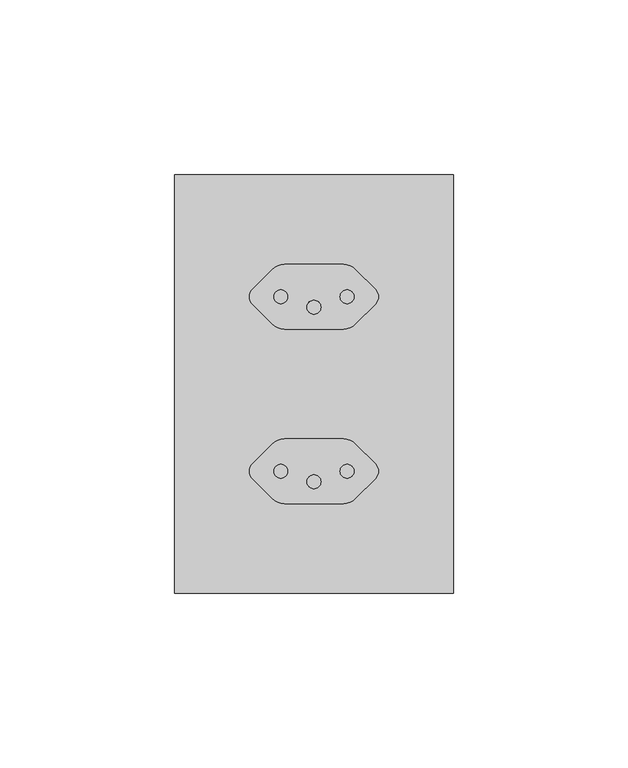
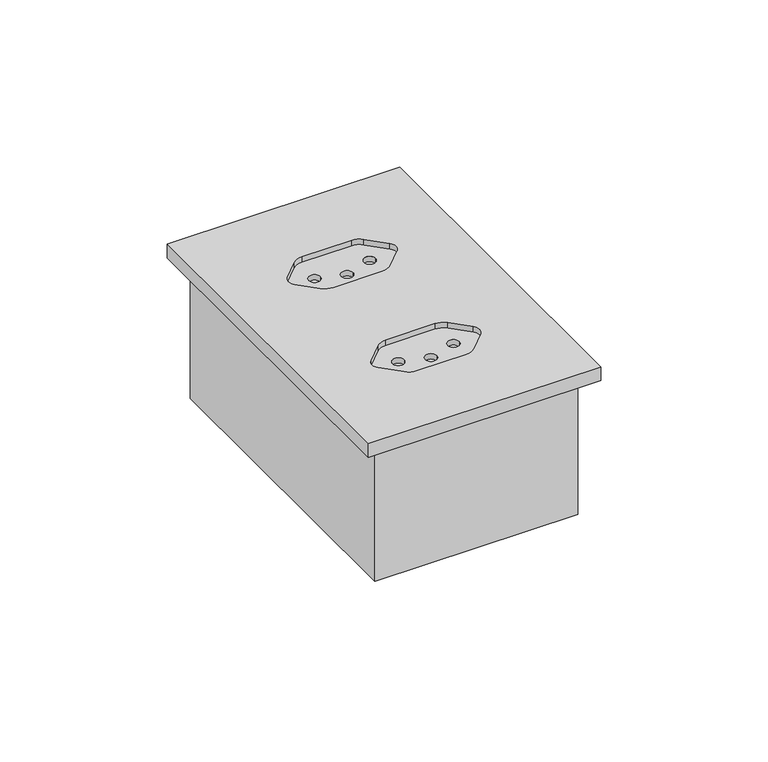
"""IFC4 building model written with IfcOpenShell, lengths in millimetres: proxy geometry, CAIXA VERTICE V7 : Tomada 10A 2s."""

from ifc_helpers import new_model, si_unit, frame, origin, place, context, project, spatial, polyline, circle_curve, faceted_brep, source, transform, mapped, element, save
from ifc_brep_helpers import plane_surface, revolved_surface, advanced_brep


def electrical_fixtures_dab928c3(model_context):
    return source(origin(), model_context, "Body", "SolidModel", [
        faceted_brep([(33.0, -1047.0, -48.0), (-33.0, -1047.0, -48.0), (-33.0, -1153.0, -48.0), (33.0, -1153.0, -48.0), (35.0, -1155.0, -50.0), (-35.0, -1155.0, -50.0), (-35.0, -1045.0, -50.0), (35.0, -1045.0, -50.0), (35.0, -1155.0, 0.0), (-35.0, -1155.0, 0.0), (-35.0, -1045.0, 0.0), (35.0, -1045.0, 0.0), (33.0, -1153.0, 0.0), (-33.0, -1153.0, 0.0), (-33.0, -1047.0, 0.0), (33.0, -1047.0, 0.0)], [[[0, 1, 2, 3]], [[4, 5, 6, 7]], [[4, 8, 9, 5]], [[9, 10, 6, 5]], [[10, 11, 7, 6]], [[11, 8, 4, 7]], [[8, 11, 10, 9], [12, 13, 14, 15]], [[15, 0, 3, 12]], [[14, 1, 0, 15]], [[13, 2, 1, 14]], [[12, 3, 2, 13]]]),
        advanced_brep(
        [(40.0, -1160.0, 5.0), (40.0, -1040.0, 5.0), (-40.0, -1040.0, 5.0), (-40.0, -1160.0, 5.0), (8.4215729, -1115.75, 5.0), (11.9571068, -1117.2144661, 5.0), (17.6213203, -1122.8786797, 5.0), (17.6213203, -1127.1213203, 5.0), (11.9571068, -1132.7855339, 5.0), (8.4215729, -1134.25, 5.0), (-8.4215729, -1134.25, 5.0), (-11.9571068, -1132.7855339, 5.0), (-17.6213203, -1127.1213203, 5.0), (-17.6213203, -1122.8786797, 5.0), (-11.9571068, -1117.2144661, 5.0), (-8.4215729, -1115.75, 5.0), (8.4215729, -1065.75, 5.0), (11.9571068, -1067.2144661, 5.0), (17.6213203, -1072.8786797, 5.0), (17.6213203, -1077.1213203, 5.0), (11.9571068, -1082.7855339, 5.0), (8.4215729, -1084.25, 5.0), (-8.4215729, -1084.25, 5.0), (-11.9571068, -1082.7855339, 5.0), (-17.6213203, -1077.1213203, 5.0), (-17.6213203, -1072.8786797, 5.0), (-11.9571068, -1067.2144661, 5.0), (-8.4215729, -1065.75, 5.0), (-40.0, -1160.0, 0.0), (-40.0, -1040.0, 0.0), (40.0, -1040.0, 0.0), (40.0, -1160.0, 0.0), (8.4215729, -1115.75, 3.0), (-8.4215729, -1115.75, 3.0), (-11.9571068, -1117.2144661, 3.0), (-17.6213203, -1122.8786797, 3.0), (-17.6213203, -1127.1213203, 3.0), (-11.9571068, -1132.7855339, 3.0), (-8.4215729, -1134.25, 3.0), (8.4215729, -1134.25, 3.0), (11.9571068, -1132.7855339, 3.0), (17.6213203, -1127.1213203, 3.0), (17.6213203, -1122.8786797, 3.0), (11.9571068, -1117.2144661, 3.0), (-7.5, -1125.0, 3.0), (-11.5, -1125.0, 3.0), (11.5, -1125.0, 3.0), (7.5, -1125.0, 3.0), (2.0, -1128.0, 3.0), (-2.0, -1128.0, 3.0), (-11.5, -1125.0, 1.0), (-7.5, -1125.0, 1.0), (7.5, -1125.0, 1.0), (11.5, -1125.0, 1.0), (-2.0, -1128.0, 1.0), (2.0, -1128.0, 1.0), (8.4215729, -1065.75, 3.0), (-8.4215729, -1065.75, 3.0), (-11.9571068, -1067.2144661, 3.0), (-17.6213203, -1072.8786797, 3.0), (-17.6213203, -1077.1213203, 3.0), (-11.9571068, -1082.7855339, 3.0), (-8.4215729, -1084.25, 3.0), (8.4215729, -1084.25, 3.0), (11.9571068, -1082.7855339, 3.0), (17.6213203, -1077.1213203, 3.0), (17.6213203, -1072.8786797, 3.0), (11.9571068, -1067.2144661, 3.0), (-7.5, -1075.0, 3.0), (-11.5, -1075.0, 3.0), (11.5, -1075.0, 3.0), (7.5, -1075.0, 3.0), (2.0, -1078.0, 3.0), (-2.0, -1078.0, 3.0), (-11.5, -1075.0, 1.0), (-7.5, -1075.0, 1.0), (7.5, -1075.0, 1.0), (11.5, -1075.0, 1.0), (-2.0, -1078.0, 1.0), (2.0, -1078.0, 1.0)],
        [
            (0, 1),
            (1, 2),
            (2, 3),
            (3, 0),
            (4, 5, circle_curve(frame((8.4215729, -1120.75, 5.0), z_axis=(0.0, 0.0, -1.0), x_axis=(-1.0, 0.0, 0.0)), 5.0)),
            (5, 6),
            (6, 7, circle_curve(frame((15.5, -1125.0, 5.0), z_axis=(0.0, 0.0, -1.0), x_axis=(-1.0, 0.0, 0.0)), 3.0)),
            (7, 8),
            (8, 9, circle_curve(frame((8.4215729, -1129.25, 5.0), z_axis=(0.0, 0.0, -1.0), x_axis=(-1.0, 0.0, 0.0)), 5.0)),
            (9, 10),
            (10, 11, circle_curve(frame((-8.4215729, -1129.25, 5.0), z_axis=(0.0, 0.0, -1.0), x_axis=(-1.0, 0.0, 0.0)), 5.0)),
            (11, 12),
            (12, 13, circle_curve(frame((-15.5, -1125.0, 5.0), z_axis=(0.0, 0.0, -1.0), x_axis=(-1.0, 0.0, 0.0)), 3.0)),
            (13, 14),
            (14, 15, circle_curve(frame((-8.4215729, -1120.75, 5.0), z_axis=(0.0, 0.0, -1.0), x_axis=(-1.0, 0.0, 0.0)), 5.0)),
            (15, 4),
            (16, 17, circle_curve(frame((8.4215729, -1070.75, 5.0), z_axis=(0.0, 0.0, -1.0), x_axis=(-1.0, 0.0, 0.0)), 5.0)),
            (17, 18),
            (18, 19, circle_curve(frame((15.5, -1075.0, 5.0), z_axis=(0.0, 0.0, -1.0), x_axis=(-1.0, 0.0, 0.0)), 3.0)),
            (19, 20),
            (20, 21, circle_curve(frame((8.4215729, -1079.25, 5.0), z_axis=(0.0, 0.0, -1.0), x_axis=(-1.0, 0.0, 0.0)), 5.0)),
            (21, 22),
            (22, 23, circle_curve(frame((-8.4215729, -1079.25, 5.0), z_axis=(0.0, 0.0, -1.0), x_axis=(-1.0, 0.0, 0.0)), 5.0)),
            (23, 24),
            (24, 25, circle_curve(frame((-15.5, -1075.0, 5.0), z_axis=(0.0, 0.0, -1.0), x_axis=(-1.0, 0.0, 0.0)), 3.0)),
            (25, 26),
            (26, 27, circle_curve(frame((-8.4215729, -1070.75, 5.0), z_axis=(0.0, 0.0, -1.0), x_axis=(-1.0, 0.0, 0.0)), 5.0)),
            (27, 16),
            (28, 29),
            (29, 30),
            (30, 31),
            (31, 28),
            (3, 28),
            (31, 0),
            (2, 29),
            (1, 30),
            (32, 33),
            (33, 34, circle_curve(frame((-8.4215729, -1120.75, 3.0), z_axis=(0.0, 0.0, 1.0), x_axis=(-1.0, 0.0, 0.0)), 5.0)),
            (34, 35),
            (35, 36, circle_curve(frame((-15.5, -1125.0, 3.0), z_axis=(0.0, 0.0, 1.0), x_axis=(-1.0, 0.0, 0.0)), 3.0)),
            (36, 37),
            (37, 38, circle_curve(frame((-8.4215729, -1129.25, 3.0), z_axis=(0.0, 0.0, 1.0), x_axis=(-1.0, 0.0, 0.0)), 5.0)),
            (38, 39),
            (39, 40, circle_curve(frame((8.4215729, -1129.25, 3.0), z_axis=(0.0, 0.0, 1.0), x_axis=(-1.0, 0.0, 0.0)), 5.0)),
            (40, 41),
            (41, 42, circle_curve(frame((15.5, -1125.0, 3.0), z_axis=(0.0, 0.0, 1.0), x_axis=(-1.0, 0.0, 0.0)), 3.0)),
            (42, 43),
            (43, 32, circle_curve(frame((8.4215729, -1120.75, 3.0), z_axis=(0.0, 0.0, 1.0), x_axis=(-1.0, 0.0, 0.0)), 5.0)),
            (44, 45, circle_curve(frame((-9.5, -1125.0, 3.0), z_axis=(0.0, 0.0, -1.0), x_axis=(1.0, -2.301812013077709e-12, 0.0)), 2.0)),
            (45, 44, circle_curve(frame((-9.5, -1125.0, 3.0), z_axis=(0.0, 0.0, -1.0), x_axis=(1.0, -2.301812013077709e-12, 0.0)), 2.0)),
            (46, 47, circle_curve(frame((9.5, -1125.0, 3.0), z_axis=(0.0, 0.0, -1.0), x_axis=(1.0, -2.301812013077709e-12, 0.0)), 2.0)),
            (47, 46, circle_curve(frame((9.5, -1125.0, 3.0), z_axis=(0.0, 0.0, -1.0), x_axis=(1.0, -2.301812013077709e-12, 0.0)), 2.0)),
            (48, 49, circle_curve(frame((0.0, -1128.0, 3.0), z_axis=(0.0, 0.0, -1.0), x_axis=(1.0, -2.301812013077709e-12, 0.0)), 2.0)),
            (49, 48, circle_curve(frame((0.0, -1128.0, 3.0), z_axis=(0.0, 0.0, -1.0), x_axis=(1.0, -2.301812013077709e-12, 0.0)), 2.0)),
            (32, 4),
            (15, 33),
            (14, 34),
            (13, 35),
            (12, 36),
            (11, 37),
            (10, 38),
            (9, 39),
            (8, 40),
            (7, 41),
            (6, 42),
            (5, 43),
            (50, 51, circle_curve(frame((-9.5, -1125.0, 1.0), z_axis=(0.0, 0.0, 1.0), x_axis=(1.0, -2.301812013077709e-12, 0.0)), 2.0)),
            (51, 50, circle_curve(frame((-9.5, -1125.0, 1.0), z_axis=(0.0, 0.0, 1.0), x_axis=(1.0, -2.301812013077709e-12, 0.0)), 2.0)),
            (52, 53, circle_curve(frame((9.5, -1125.0, 1.0), z_axis=(0.0, 0.0, 1.0), x_axis=(1.0, -2.301812013077709e-12, 0.0)), 2.0)),
            (53, 52, circle_curve(frame((9.5, -1125.0, 1.0), z_axis=(0.0, 0.0, 1.0), x_axis=(1.0, -2.301812013077709e-12, 0.0)), 2.0)),
            (54, 55, circle_curve(frame((0.0, -1128.0, 1.0), z_axis=(0.0, 0.0, 1.0), x_axis=(1.0, -2.301812013077709e-12, 0.0)), 2.0)),
            (55, 54, circle_curve(frame((0.0, -1128.0, 1.0), z_axis=(0.0, 0.0, 1.0), x_axis=(1.0, -2.301812013077709e-12, 0.0)), 2.0)),
            (45, 50),
            (51, 44),
            (47, 52),
            (53, 46),
            (49, 54),
            (55, 48),
            (56, 57),
            (57, 58, circle_curve(frame((-8.4215729, -1070.75, 3.0), z_axis=(0.0, 0.0, 1.0), x_axis=(-1.0, 0.0, 0.0)), 5.0)),
            (58, 59),
            (59, 60, circle_curve(frame((-15.5, -1075.0, 3.0), z_axis=(0.0, 0.0, 1.0), x_axis=(-1.0, 0.0, 0.0)), 3.0)),
            (60, 61),
            (61, 62, circle_curve(frame((-8.4215729, -1079.25, 3.0), z_axis=(0.0, 0.0, 1.0), x_axis=(-1.0, 0.0, 0.0)), 5.0)),
            (62, 63),
            (63, 64, circle_curve(frame((8.4215729, -1079.25, 3.0), z_axis=(0.0, 0.0, 1.0), x_axis=(-1.0, 0.0, 0.0)), 5.0)),
            (64, 65),
            (65, 66, circle_curve(frame((15.5, -1075.0, 3.0), z_axis=(0.0, 0.0, 1.0), x_axis=(-1.0, 0.0, 0.0)), 3.0)),
            (66, 67),
            (67, 56, circle_curve(frame((8.4215729, -1070.75, 3.0), z_axis=(0.0, 0.0, 1.0), x_axis=(-1.0, 0.0, 0.0)), 5.0)),
            (68, 69, circle_curve(frame((-9.5, -1075.0, 3.0), z_axis=(0.0, 0.0, -1.0), x_axis=(1.0, -2.301812013077709e-12, 0.0)), 2.0)),
            (69, 68, circle_curve(frame((-9.5, -1075.0, 3.0), z_axis=(0.0, 0.0, -1.0), x_axis=(1.0, -2.301812013077709e-12, 0.0)), 2.0)),
            (70, 71, circle_curve(frame((9.5, -1075.0, 3.0), z_axis=(0.0, 0.0, -1.0), x_axis=(1.0, -2.301812013077709e-12, 0.0)), 2.0)),
            (71, 70, circle_curve(frame((9.5, -1075.0, 3.0), z_axis=(0.0, 0.0, -1.0), x_axis=(1.0, -2.301812013077709e-12, 0.0)), 2.0)),
            (72, 73, circle_curve(frame((0.0, -1078.0, 3.0), z_axis=(0.0, 0.0, -1.0), x_axis=(1.0, -2.301812013077709e-12, 0.0)), 2.0)),
            (73, 72, circle_curve(frame((0.0, -1078.0, 3.0), z_axis=(0.0, 0.0, -1.0), x_axis=(1.0, -2.301812013077709e-12, 0.0)), 2.0)),
            (56, 16),
            (27, 57),
            (26, 58),
            (25, 59),
            (24, 60),
            (23, 61),
            (22, 62),
            (21, 63),
            (20, 64),
            (19, 65),
            (18, 66),
            (17, 67),
            (74, 75, circle_curve(frame((-9.5, -1075.0, 1.0), z_axis=(0.0, 0.0, 1.0), x_axis=(1.0, -2.301812013077709e-12, 0.0)), 2.0)),
            (75, 74, circle_curve(frame((-9.5, -1075.0, 1.0), z_axis=(0.0, 0.0, 1.0), x_axis=(1.0, -2.301812013077709e-12, 0.0)), 2.0)),
            (76, 77, circle_curve(frame((9.5, -1075.0, 1.0), z_axis=(0.0, 0.0, 1.0), x_axis=(1.0, -2.301812013077709e-12, 0.0)), 2.0)),
            (77, 76, circle_curve(frame((9.5, -1075.0, 1.0), z_axis=(0.0, 0.0, 1.0), x_axis=(1.0, -2.301812013077709e-12, 0.0)), 2.0)),
            (78, 79, circle_curve(frame((0.0, -1078.0, 1.0), z_axis=(0.0, 0.0, 1.0), x_axis=(1.0, -2.301812013077709e-12, 0.0)), 2.0)),
            (79, 78, circle_curve(frame((0.0, -1078.0, 1.0), z_axis=(0.0, 0.0, 1.0), x_axis=(1.0, -2.301812013077709e-12, 0.0)), 2.0)),
            (69, 74),
            (75, 68),
            (71, 76),
            (77, 70),
            (73, 78),
            (79, 72),
        ],
        [
            plane_surface(frame((-60.0, -1160.0, 5.0), z_axis=(0.0, 0.0, 1.0), x_axis=(-1.0, 0.0, 0.0))),
            plane_surface(frame((-60.0, -1160.0, 0.0), z_axis=(0.0, 0.0, -1.0), x_axis=(1.0, 0.0, 0.0))),
            plane_surface(frame((40.0, -1160.0, 5.0), z_axis=(0.0, -1.0, 0.0), x_axis=(0.0, 0.0, -1.0))),
            plane_surface(frame((-40.0, -1160.0, 5.0), z_axis=(-1.0, 0.0, 0.0), x_axis=(0.0, 0.0, -1.0))),
            plane_surface(frame((-40.0, -1040.0, 5.0), z_axis=(0.0, 1.0, 0.0), x_axis=(0.0, 0.0, -1.0))),
            plane_surface(frame((40.0, -1040.0, 5.0), z_axis=(1.0, 0.0, 0.0), x_axis=(0.0, 0.0, -1.0))),
            plane_surface(frame((3.4215729, -1120.75, 3.0), z_axis=(0.0, 0.0, 1.0), x_axis=(0.0, -1.0, 0.0))),
            plane_surface(frame((-8.4215729, -1115.75, 5.0), z_axis=(0.0, -1.0, 0.0), x_axis=(0.0, 0.0, -1.0))),
            revolved_surface(polyline([(-13.4215729, -1120.75, 5.0), (-13.4215729, -1120.75, 3.0)]), (-8.4215729, -1120.75, 3.0), (0.0, 0.0, 1.0)),
            plane_surface(frame((-17.6213203, -1122.8786797, 5.0), z_axis=(0.7071067811865045, -0.7071067811865905, 0.0), x_axis=(0.0, 0.0, -1.0))),
            revolved_surface(polyline([(-18.5, -1125.0, 5.0), (-18.5, -1125.0, 3.0)]), (-15.5, -1125.0, 3.0), (0.0, 0.0, 1.0)),
            plane_surface(frame((-11.9571068, -1132.7855339, 5.0), z_axis=(0.7071067811865515, 0.7071067811865437, 0.0), x_axis=(0.0, 0.0, -1.0))),
            revolved_surface(polyline([(-13.4215729, -1129.25, 5.0), (-13.4215729, -1129.25, 3.0)]), (-8.4215729, -1129.25, 3.0), (0.0, 0.0, 1.0)),
            plane_surface(frame((8.4215729, -1134.25, 5.0), z_axis=(0.0, 1.0, 0.0), x_axis=(0.0, 0.0, -1.0))),
            revolved_surface(polyline([(3.4215728999999993, -1129.25, 5.0), (3.4215728999999993, -1129.25, 3.0)]), (8.4215729, -1129.25, 3.0), (0.0, 0.0, 1.0)),
            plane_surface(frame((17.6213203, -1127.1213203, 5.0), z_axis=(-0.7071067811865307, 0.7071067811865643, 0.0), x_axis=(0.0, 0.0, -1.0))),
            revolved_surface(polyline([(12.5, -1125.0, 5.0), (12.5, -1125.0, 3.0)]), (15.5, -1125.0, 3.0), (0.0, 0.0, 1.0)),
            plane_surface(frame((11.9571068, -1117.2144661, 5.0), z_axis=(-0.7071067811865893, -0.7071067811865058, 0.0), x_axis=(0.0, 0.0, -1.0))),
            revolved_surface(polyline([(3.4215728999999993, -1120.75, 5.0), (3.4215728999999993, -1120.75, 3.0)]), (8.4215729, -1120.75, 3.0), (0.0, 0.0, 1.0)),
            plane_surface(frame((-7.5, -1125.0, 1.0), z_axis=(0.0, 0.0, 1.0), x_axis=(2.301812013077709e-12, 1.0, 0.0))),
            revolved_surface(polyline([(-7.5, -1125.0000000000045, 3.0), (-7.5, -1125.0000000000045, 1.0)]), (-9.5, -1125.0, 1.0), (0.0, 0.0, 1.0)),
            revolved_surface(polyline([(11.5, -1125.0000000000045, 3.0), (11.5, -1125.0000000000045, 1.0)]), (9.5, -1125.0, 5.0), (0.0, 0.0, 1.0)),
            revolved_surface(polyline([(2.0, -1128.0000000000045, 3.0), (2.0, -1128.0000000000045, 1.0)]), (0.0, -1128.0, 5.0), (0.0, 0.0, 1.0)),
            plane_surface(frame((3.4215729, -1070.75, 3.0), z_axis=(0.0, 0.0, 1.0), x_axis=(0.0, -1.0, 0.0))),
            plane_surface(frame((-8.4215729, -1065.75, 5.0), z_axis=(0.0, -1.0, 0.0), x_axis=(0.0, 0.0, -1.0))),
            revolved_surface(polyline([(-13.4215729, -1070.75, 5.0), (-13.4215729, -1070.75, 3.0)]), (-8.4215729, -1070.75, 3.0), (0.0, 0.0, 1.0)),
            plane_surface(frame((-17.6213203, -1072.8786797, 5.0), z_axis=(0.7071067811865045, -0.7071067811865905, 0.0), x_axis=(0.0, 0.0, -1.0))),
            revolved_surface(polyline([(-18.5, -1075.0, 5.0), (-18.5, -1075.0, 3.0)]), (-15.5, -1075.0, 3.0), (0.0, 0.0, 1.0)),
            plane_surface(frame((-11.9571068, -1082.7855339, 5.0), z_axis=(0.7071067811865515, 0.7071067811865437, 0.0), x_axis=(0.0, 0.0, -1.0))),
            revolved_surface(polyline([(-13.4215729, -1079.25, 5.0), (-13.4215729, -1079.25, 3.0)]), (-8.4215729, -1079.25, 3.0), (0.0, 0.0, 1.0)),
            plane_surface(frame((8.4215729, -1084.25, 5.0), z_axis=(0.0, 1.0, 0.0), x_axis=(0.0, 0.0, -1.0))),
            revolved_surface(polyline([(3.4215728999999993, -1079.25, 5.0), (3.4215728999999993, -1079.25, 3.0)]), (8.4215729, -1079.25, 3.0), (0.0, 0.0, 1.0)),
            plane_surface(frame((17.6213203, -1077.1213203, 5.0), z_axis=(-0.7071067811865307, 0.7071067811865643, 0.0), x_axis=(0.0, 0.0, -1.0))),
            revolved_surface(polyline([(12.5, -1075.0, 5.0), (12.5, -1075.0, 3.0)]), (15.5, -1075.0, 3.0), (0.0, 0.0, 1.0)),
            plane_surface(frame((11.9571068, -1067.2144661, 5.0), z_axis=(-0.7071067811865893, -0.7071067811865058, 0.0), x_axis=(0.0, 0.0, -1.0))),
            revolved_surface(polyline([(3.4215728999999993, -1070.75, 5.0), (3.4215728999999993, -1070.75, 3.0)]), (8.4215729, -1070.75, 3.0), (0.0, 0.0, 1.0)),
            plane_surface(frame((-7.5, -1075.0, 1.0), z_axis=(0.0, 0.0, 1.0), x_axis=(2.301812013077709e-12, 1.0, 0.0))),
            revolved_surface(polyline([(-7.5, -1075.0000000000045, 3.0), (-7.5, -1075.0000000000045, 1.0)]), (-9.5, -1075.0, 1.0), (0.0, 0.0, 1.0)),
            revolved_surface(polyline([(11.5, -1075.0000000000045, 3.0), (11.5, -1075.0000000000045, 1.0)]), (9.5, -1075.0, 5.0), (0.0, 0.0, 1.0)),
            revolved_surface(polyline([(2.0, -1078.0000000000045, 3.0), (2.0, -1078.0000000000045, 1.0)]), (0.0, -1078.0, 5.0), (0.0, 0.0, 1.0)),
        ],
        [
            (0, [[1, 2, 3, 4], [5, 6, 7, 8, 9, 10, 11, 12, 13, 14, 15, 16], [17, 18, 19, 20, 21, 22, 23, 24, 25, 26, 27, 28]]),
            (1, [[29, 30, 31, 32]]),
            (2, [[33, -32, 34, -4]]),
            (3, [[35, -29, -33, -3]]),
            (4, [[36, -30, -35, -2]]),
            (5, [[-34, -31, -36, -1]]),
            (6, [[37, 38, 39, 40, 41, 42, 43, 44, 45, 46, 47, 48], [49, 50], [51, 52], [53, 54]]),
            (7, [[55, -16, 56, -37]]),
            (8, [[-56, -15, 57, -38]]),
            (9, [[-57, -14, 58, -39]]),
            (10, [[-58, -13, 59, -40]]),
            (11, [[-59, -12, 60, -41]]),
            (12, [[-60, -11, 61, -42]]),
            (13, [[-61, -10, 62, -43]]),
            (14, [[-62, -9, 63, -44]]),
            (15, [[-63, -8, 64, -45]]),
            (16, [[-64, -7, 65, -46]]),
            (17, [[-65, -6, 66, -47]]),
            (18, [[-66, -5, -55, -48]]),
            (19, [[67, 68]]),
            (19, [[69, 70]]),
            (19, [[71, 72]]),
            (20, [[73, -68, 74, -50]]),
            (20, [[-74, -67, -73, -49]]),
            (21, [[75, -70, 76, -52]]),
            (21, [[-76, -69, -75, -51]]),
            (22, [[77, -72, 78, -54]]),
            (22, [[-78, -71, -77, -53]]),
            (23, [[79, 80, 81, 82, 83, 84, 85, 86, 87, 88, 89, 90], [91, 92], [93, 94], [95, 96]]),
            (24, [[97, -28, 98, -79]]),
            (25, [[-98, -27, 99, -80]]),
            (26, [[-99, -26, 100, -81]]),
            (27, [[-100, -25, 101, -82]]),
            (28, [[-101, -24, 102, -83]]),
            (29, [[-102, -23, 103, -84]]),
            (30, [[-103, -22, 104, -85]]),
            (31, [[-104, -21, 105, -86]]),
            (32, [[-105, -20, 106, -87]]),
            (33, [[-106, -19, 107, -88]]),
            (34, [[-107, -18, 108, -89]]),
            (35, [[-108, -17, -97, -90]]),
            (36, [[109, 110]]),
            (36, [[111, 112]]),
            (36, [[113, 114]]),
            (37, [[115, -110, 116, -92]]),
            (37, [[-116, -109, -115, -91]]),
            (38, [[117, -112, 118, -94]]),
            (38, [[-118, -111, -117, -93]]),
            (39, [[119, -114, 120, -96]]),
            (39, [[-120, -113, -119, -95]]),
        ],
    ),
    ])


if __name__ == "__main__":
    model = new_model("IFC4")
    model_context = context("Model", 3, world=origin())
    ifc_project = project(units=[si_unit("LENGTHUNIT", "METRE", prefix="MILLI")], contexts=[model_context])
    site = spatial("IfcSite", under=ifc_project)
    building = spatial("IfcBuilding", under=site)
    placement = place(None, origin())
    electrical_fixtures_shape = electrical_fixtures_dab928c3(model_context)
    element("IfcBuildingElementProxy", 1, Name="CAIXA VERTICE V7 : Tomada 10A 2s", ObjectType="CAIXA VERTICE V7 : Tomada 10A 2s", at=placement, inside=building, context=model_context, shape_type="MappedRepresentation", body=[
        mapped(electrical_fixtures_shape, transform((0.0, 0.0, 0.0), x_axis=(1.0, 0.0, 0.0), y_axis=(0.0, 1.0, 0.0), z_axis=(0.0, 0.0, 1.0))),
    ])
    save(model, "model.ifc")

# Revit data of these elements
# Type "CAIXA VERTICE V7 : Tomada 10A 2s"
#   URL = "www.facebook.com/verticetreinamentos"
#   SEÇÃO [instance default] = ""
#   Rotação [instance default] = 0.00°
#   LARGURA DA TAMPA = 0.08 m
#   BORDA = 0.01 m
#   ALTURA DE INSTALAÇÃO [instance default] = 1.10 m
#   Distância Anotação [instance default] = 0.0015 m
#   ALTURA DA TAMPA = 0.12 m
#   Vertical [instance default] = yes
#   VER SEÇÃO [instance default] = no
#   SHADE ESQ [instance default] = no
#   SHADE DIR [instance default] = yes
#   HORIZONTAL [instance default] = no
#   ANDAR COM A LEGENDA [instance default] = 0
#   Material Tampa [instance default] = Plástico, branco opaco
#   Caixa = element 1798515
#   Anotação = element 1798529
#   Default Elevation = 0
# Element 1 (IfcBuildingElementProxy, "CAIXA VERTICE V7 : Tomada 10A 2s")
#   VER SEÇÃO = yes
#   Materials on its faces: "Plástico, branco opaco"
# Materials
#   "Plástico, branco opaco": class "Plástico", colour RGB 120 120 120, transparency 0, Description = "Plastic, generic, opaque white", Cost = 0
